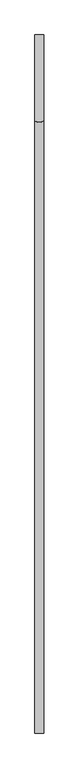
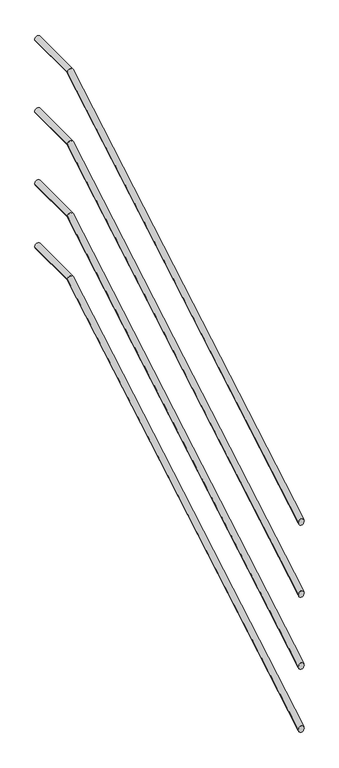
"""IFC4 building model written with IfcOpenShell, lengths in millimetres: railing geometry."""

from ifc_helpers import new_model, si_unit, frame, origin, place, context, project, spatial, circle_curve, ellipse_curve, source, transform, mapped, element, save
from ifc_brep_helpers import plane_surface, cylinder_surface, advanced_brep


def railing_ea222afd(model_context):
    return source(origin(), model_context, "Body", "AdvancedBrep", [
        advanced_brep(
        [(-3259.6, 13399.5208589, 7257.5963084), (-3289.6, 13399.5208589, 7257.5963084), (-3259.6, 15503.576096, 8484.9618634), (-3289.6, 15503.576096, 8484.9618634), (-3259.6, 15799.5208589, 8484.9618634), (-3289.6, 15799.5208589, 8484.9618634)],
        [
            (0, 1, ellipse_curve(frame((-3274.6, 13399.5208589, 7257.5963084), z_axis=(0.0, -1.0, 0.0), x_axis=(0.0, 0.0, -1.0)), 17.365555, 15.0)),
            (1, 0, ellipse_curve(frame((-3274.6, 13399.5208589, 7257.5963084), z_axis=(0.0, -1.0, 0.0), x_axis=(0.0, 0.0, -1.0)), 17.365555, 15.0)),
            (0, 2),
            (2, 3, ellipse_curve(frame((-3274.6, 15503.576096, 8484.9618634), z_axis=(0.0, -0.9653442134540492, -0.26097997921446614), x_axis=(0.0, 0.26097997921446614, -0.9653442134540491)), 15.5384989, 15.0)),
            (3, 1),
            (3, 2, ellipse_curve(frame((-3274.6, 15503.576096, 8484.9618634), z_axis=(0.0, -0.9653442134540492, -0.26097997921446614), x_axis=(0.0, 0.26097997921446614, -0.9653442134540491)), 15.5384989, 15.0)),
            (4, 5, circle_curve(frame((-3274.6, 15799.5208589, 8484.9618634), z_axis=(0.0, 1.0, 0.0), x_axis=(-1.0, 0.0, 0.0)), 15.0)),
            (5, 4, circle_curve(frame((-3274.6, 15799.5208589, 8484.9618634), z_axis=(0.0, 1.0, 0.0), x_axis=(-1.0, 0.0, 0.0)), 15.0)),
            (2, 4),
            (5, 3),
        ],
        [
            plane_surface(frame((-3274.6, 13399.5208589, 7274.9618634), z_axis=(0.0, -1.0, 0.0), x_axis=(0.0, 0.0, 1.0))),
            cylinder_surface(frame((-3274.6, 13407.0789243, 7262.0051799), z_axis=(0.0, -0.8637789008984336, -0.5038710255240859), x_axis=(-1.0, 0.0, 0.0)), 15.0),
            plane_surface(frame((-3274.6, 15799.5208589, 8499.9618634), z_axis=(0.0, 1.0, 0.0), x_axis=(0.0, 0.0, 1.0))),
            cylinder_surface(frame((-3274.6, 15499.5208589, 8484.9618634), z_axis=(0.0, -1.0, 0.0), x_axis=(-1.0, 0.0, 0.0)), 15.0),
        ],
        [
            (0, [[1, 2]]),
            (1, [[-1, 3, 4, 5]]),
            (1, [[-2, -5, 6, -3]]),
            (2, [[7, 8]]),
            (3, [[-4, 9, -8, 10]]),
            (3, [[-6, -10, -7, -9]]),
        ],
    ),
        advanced_brep(
        [(-3259.6, 13399.5208589, 6457.5963084), (-3289.6, 13399.5208589, 6457.5963084), (-3259.6, 15503.576096, 7684.9618634), (-3289.6, 15503.576096, 7684.9618634), (-3259.6, 15799.5208589, 7684.9618634), (-3289.6, 15799.5208589, 7684.9618634)],
        [
            (0, 1, ellipse_curve(frame((-3274.6, 13399.5208589, 6457.5963084), z_axis=(0.0, -1.0, 0.0), x_axis=(0.0, 0.0, -1.0)), 17.365555, 15.0)),
            (1, 0, ellipse_curve(frame((-3274.6, 13399.5208589, 6457.5963084), z_axis=(0.0, -1.0, 0.0), x_axis=(0.0, 0.0, -1.0)), 17.365555, 15.0)),
            (0, 2),
            (2, 3, ellipse_curve(frame((-3274.6, 15503.576096, 7684.9618634), z_axis=(0.0, -0.9653442134540492, -0.26097997921446614), x_axis=(0.0, 0.26097997921446614, -0.9653442134540491)), 15.5384989, 15.0)),
            (3, 1),
            (3, 2, ellipse_curve(frame((-3274.6, 15503.576096, 7684.9618634), z_axis=(0.0, -0.9653442134540492, -0.26097997921446614), x_axis=(0.0, 0.26097997921446614, -0.9653442134540491)), 15.5384989, 15.0)),
            (4, 5, circle_curve(frame((-3274.6, 15799.5208589, 7684.9618634), z_axis=(0.0, 1.0, 0.0), x_axis=(-1.0, 0.0, 0.0)), 15.0)),
            (5, 4, circle_curve(frame((-3274.6, 15799.5208589, 7684.9618634), z_axis=(0.0, 1.0, 0.0), x_axis=(-1.0, 0.0, 0.0)), 15.0)),
            (2, 4),
            (5, 3),
        ],
        [
            plane_surface(frame((-3274.6, 13399.5208589, 6474.9618634), z_axis=(0.0, -1.0, 0.0), x_axis=(0.0, 0.0, 1.0))),
            cylinder_surface(frame((-3274.6, 13407.0789243, 6462.0051799), z_axis=(0.0, -0.8637789008984336, -0.5038710255240859), x_axis=(-1.0, 0.0, 0.0)), 15.0),
            plane_surface(frame((-3274.6, 15799.5208589, 7699.9618634), z_axis=(0.0, 1.0, 0.0), x_axis=(0.0, 0.0, 1.0))),
            cylinder_surface(frame((-3274.6, 15499.5208589, 7684.9618634), z_axis=(0.0, -1.0, 0.0), x_axis=(-1.0, 0.0, 0.0)), 15.0),
        ],
        [
            (0, [[1, 2]]),
            (1, [[-1, 3, 4, 5]]),
            (1, [[-2, -5, 6, -3]]),
            (2, [[7, 8]]),
            (3, [[-4, 9, -8, 10]]),
            (3, [[-6, -10, -7, -9]]),
        ],
    ),
        advanced_brep(
        [(-3259.6, 13399.5208589, 6857.5963084), (-3289.6, 13399.5208589, 6857.5963084), (-3259.6, 15503.576096, 8084.9618634), (-3289.6, 15503.576096, 8084.9618634), (-3259.6, 15799.5208589, 8084.9618634), (-3289.6, 15799.5208589, 8084.9618634)],
        [
            (0, 1, ellipse_curve(frame((-3274.6, 13399.5208589, 6857.5963084), z_axis=(0.0, -1.0, 0.0), x_axis=(0.0, 0.0, -1.0)), 17.365555, 15.0)),
            (1, 0, ellipse_curve(frame((-3274.6, 13399.5208589, 6857.5963084), z_axis=(0.0, -1.0, 0.0), x_axis=(0.0, 0.0, -1.0)), 17.365555, 15.0)),
            (0, 2),
            (2, 3, ellipse_curve(frame((-3274.6, 15503.576096, 8084.9618634), z_axis=(0.0, -0.9653442134540492, -0.26097997921446614), x_axis=(0.0, 0.26097997921446614, -0.9653442134540491)), 15.5384989, 15.0)),
            (3, 1),
            (3, 2, ellipse_curve(frame((-3274.6, 15503.576096, 8084.9618634), z_axis=(0.0, -0.9653442134540492, -0.26097997921446614), x_axis=(0.0, 0.26097997921446614, -0.9653442134540491)), 15.5384989, 15.0)),
            (4, 5, circle_curve(frame((-3274.6, 15799.5208589, 8084.9618634), z_axis=(0.0, 1.0, 0.0), x_axis=(-1.0, 0.0, 0.0)), 15.0)),
            (5, 4, circle_curve(frame((-3274.6, 15799.5208589, 8084.9618634), z_axis=(0.0, 1.0, 0.0), x_axis=(-1.0, 0.0, 0.0)), 15.0)),
            (2, 4),
            (5, 3),
        ],
        [
            plane_surface(frame((-3274.6, 13399.5208589, 6874.9618634), z_axis=(0.0, -1.0, 0.0), x_axis=(0.0, 0.0, 1.0))),
            cylinder_surface(frame((-3274.6, 13407.0789243, 6862.0051799), z_axis=(0.0, -0.8637789008984336, -0.5038710255240859), x_axis=(-1.0, 0.0, 0.0)), 15.0),
            plane_surface(frame((-3274.6, 15799.5208589, 8099.9618634), z_axis=(0.0, 1.0, 0.0), x_axis=(0.0, 0.0, 1.0))),
            cylinder_surface(frame((-3274.6, 15499.5208589, 8084.9618634), z_axis=(0.0, -1.0, 0.0), x_axis=(-1.0, 0.0, 0.0)), 15.0),
        ],
        [
            (0, [[1, 2]]),
            (1, [[-1, 3, 4, 5]]),
            (1, [[-2, -5, 6, -3]]),
            (2, [[7, 8]]),
            (3, [[-4, 9, -8, 10]]),
            (3, [[-6, -10, -7, -9]]),
        ],
    ),
        advanced_brep(
        [(-3259.6, 13399.5208589, 6107.5963084), (-3289.6, 13399.5208589, 6107.5963084), (-3259.6, 15503.576096, 7334.9618634), (-3289.6, 15503.576096, 7334.9618634), (-3259.6, 15799.5208589, 7334.9618634), (-3289.6, 15799.5208589, 7334.9618634)],
        [
            (0, 1, ellipse_curve(frame((-3274.6, 13399.5208589, 6107.5963084), z_axis=(0.0, -1.0, 0.0), x_axis=(0.0, 0.0, -1.0)), 17.365555, 15.0)),
            (1, 0, ellipse_curve(frame((-3274.6, 13399.5208589, 6107.5963084), z_axis=(0.0, -1.0, 0.0), x_axis=(0.0, 0.0, -1.0)), 17.365555, 15.0)),
            (0, 2),
            (2, 3, ellipse_curve(frame((-3274.6, 15503.576096, 7334.9618634), z_axis=(0.0, -0.9653442134540492, -0.26097997921446614), x_axis=(0.0, 0.26097997921446614, -0.9653442134540491)), 15.5384989, 15.0)),
            (3, 1),
            (3, 2, ellipse_curve(frame((-3274.6, 15503.576096, 7334.9618634), z_axis=(0.0, -0.9653442134540492, -0.26097997921446614), x_axis=(0.0, 0.26097997921446614, -0.9653442134540491)), 15.5384989, 15.0)),
            (4, 5, circle_curve(frame((-3274.6, 15799.5208589, 7334.9618634), z_axis=(0.0, 1.0, 0.0), x_axis=(-1.0, 0.0, 0.0)), 15.0)),
            (5, 4, circle_curve(frame((-3274.6, 15799.5208589, 7334.9618634), z_axis=(0.0, 1.0, 0.0), x_axis=(-1.0, 0.0, 0.0)), 15.0)),
            (2, 4),
            (5, 3),
        ],
        [
            plane_surface(frame((-3274.6, 13399.5208589, 6124.9618634), z_axis=(0.0, -1.0, 0.0), x_axis=(0.0, 0.0, 1.0))),
            cylinder_surface(frame((-3274.6, 13407.0789243, 6112.0051799), z_axis=(0.0, -0.8637789008984336, -0.5038710255240859), x_axis=(-1.0, 0.0, 0.0)), 15.0),
            plane_surface(frame((-3274.6, 15799.5208589, 7349.9618634), z_axis=(0.0, 1.0, 0.0), x_axis=(0.0, 0.0, 1.0))),
            cylinder_surface(frame((-3274.6, 15499.5208589, 7334.9618634), z_axis=(0.0, -1.0, 0.0), x_axis=(-1.0, 0.0, 0.0)), 15.0),
        ],
        [
            (0, [[1, 2]]),
            (1, [[-1, 3, 4, 5]]),
            (1, [[-2, -5, 6, -3]]),
            (2, [[7, 8]]),
            (3, [[-4, 9, -8, 10]]),
            (3, [[-6, -10, -7, -9]]),
        ],
    ),
    ])


if __name__ == "__main__":
    model = new_model("IFC4")
    model_context = context("Model", 3, world=origin())
    ifc_project = project(units=[si_unit("LENGTHUNIT", "METRE", prefix="MILLI")], contexts=[model_context])
    site = spatial("IfcSite", under=ifc_project)
    building = spatial("IfcBuilding", under=site)
    placement = place(None, origin())
    railing_shape = railing_ea222afd(model_context)
    element("IfcRailing", 1, at=placement, inside=building, context=model_context, shape_type="MappedRepresentation", body=[
        mapped(railing_shape, transform((0.0, 0.0, 0.0), x_axis=(1.0, 0.0, 0.0), y_axis=(0.0, 1.0, 0.0), z_axis=(0.0, 0.0, 1.0))),
    ])
    save(model, "model.ifc")
